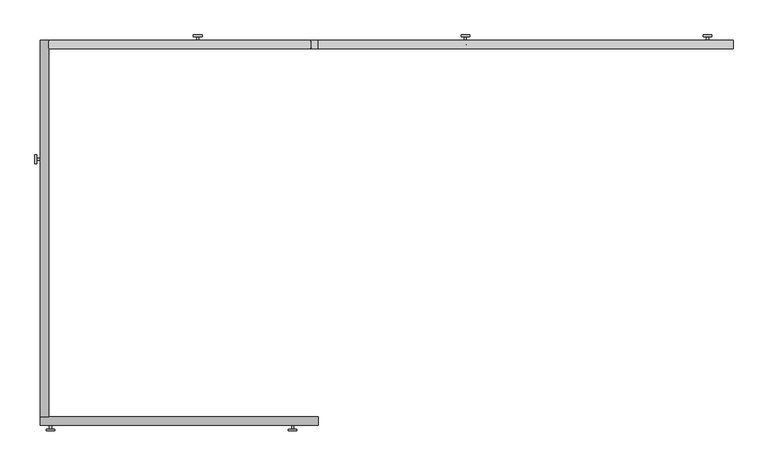
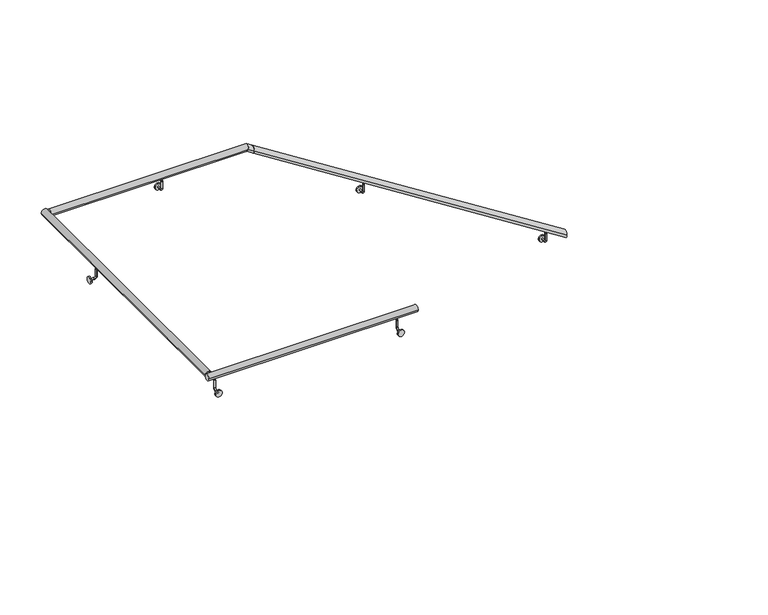
"""IFC4 building model written with IfcOpenShell, lengths in millimetres: railing geometry."""

from ifc_helpers import new_model, si_unit, point, frame, frame_2d, origin, place, context, project, spatial, circle_curve, ellipse_curve, trimmed, segment, composite_curve, outline, extrude, source, transform, mapped, element, save
from ifc_brep_helpers import plane_surface, cylinder_surface, revolved_surface, advanced_brep


def railing_9156e701(model_context):
    return source(origin(), model_context, "Body", "SolidModel", [
        advanced_brep(
        [(-47456.2877983, -5187.5461643, 4679.846421), (-47456.2877983, -5137.5461643, 4679.846421), (-49886.2877983, -5187.5461643, 6222.7035638), (-49886.2877983, -5137.5461643, 6222.7035638)],
        [
            (0, 1, ellipse_curve(frame((-47456.2877983, -5162.5461643, 4679.846421), z_axis=(1.0, 0.0, 0.0), x_axis=(0.0, 0.0, -1.0)), 29.613386, 25.0)),
            (1, 0, ellipse_curve(frame((-47456.2877983, -5162.5461643, 4679.846421), z_axis=(1.0, 0.0, 0.0), x_axis=(0.0, 0.0, -1.0)), 29.613386, 25.0)),
            (2, 3, ellipse_curve(frame((-49886.2877983, -5162.5461643, 6222.7035638), z_axis=(-1.0, 0.0, 0.0), x_axis=(0.0, 0.0, -1.0)), 29.613386, 25.0)),
            (3, 2, ellipse_curve(frame((-49886.2877983, -5162.5461643, 6222.7035638), z_axis=(-1.0, 0.0, 0.0), x_axis=(0.0, 0.0, -1.0)), 29.613386, 25.0)),
            (0, 2),
            (3, 1),
        ],
        [
            plane_surface(frame((-47456.2877983, -5162.5461643, 4709.459807), z_axis=(1.0, 0.0, 0.0), x_axis=(0.0, -1.0, 0.0))),
            plane_surface(frame((-49886.2877983, -5162.5461643, 6252.3169499), z_axis=(-1.0, 0.0, 0.0), x_axis=(0.0, -1.0, 0.0))),
            cylinder_surface(frame((-47469.6880017, -5162.5461643, 4688.3544866), z_axis=(0.8442128152478047, 0.0, -0.5360081366652713), x_axis=(0.0, 1.0, 0.0)), 25.0),
        ],
        [
            (0, [[1, 2]]),
            (1, [[3, 4]]),
            (2, [[-1, 5, -4, 6]]),
            (2, [[-2, -6, -3, -5]]),
        ],
    ),
        advanced_brep(
        [(-49886.2877983, -5187.5461643, 6222.7035638), (-49886.2877983, -5137.5461643, 6222.7035638), (-49933.6546852, -5187.5461643, 6252.7777778), (-49933.6546852, -5137.5461643, 6252.7777778), (-51463.5128792, -5187.5461643, 6252.7777778), (-51463.5128792, -5137.5461643, 6252.7777778)],
        [
            (0, 1, ellipse_curve(frame((-49886.2877983, -5162.5461643, 6222.7035638), z_axis=(1.0, 0.0, 0.0), x_axis=(0.0, 0.0, -1.0)), 29.613386, 25.0)),
            (1, 0, ellipse_curve(frame((-49886.2877983, -5162.5461643, 6222.7035638), z_axis=(1.0, 0.0, 0.0), x_axis=(0.0, 0.0, -1.0)), 29.613386, 25.0)),
            (0, 2),
            (2, 3, ellipse_curve(frame((-49933.6546852, -5162.5461643, 6252.7777778), z_axis=(0.9602637177483601, 0.0, -0.2790942356554467), x_axis=(-0.27909423565544716, 0.0, -0.9602637177483598)), 26.0345148, 25.0)),
            (3, 1),
            (3, 2, ellipse_curve(frame((-49933.6546852, -5162.5461643, 6252.7777778), z_axis=(0.9602637177483601, 0.0, -0.2790942356554467), x_axis=(-0.27909423565544716, 0.0, -0.9602637177483598)), 26.0345148, 25.0)),
            (4, 5, circle_curve(frame((-51463.5128792, -5162.5461643, 6252.7777778), z_axis=(-1.0, 0.0, 0.0), x_axis=(0.0, 1.0, 0.0)), 25.0)),
            (5, 4, circle_curve(frame((-51463.5128792, -5162.5461643, 6252.7777778), z_axis=(-1.0, 0.0, 0.0), x_axis=(0.0, 1.0, 0.0)), 25.0)),
            (2, 4),
            (5, 3),
        ],
        [
            plane_surface(frame((-49886.2877983, -5162.5461643, 6252.3169499), z_axis=(1.0, 0.0, 0.0), x_axis=(0.0, -1.0, 0.0))),
            cylinder_surface(frame((-49899.6880017, -5162.5461643, 6231.2116295), z_axis=(0.844212815247804, 0.0, -0.5360081366652724), x_axis=(0.0, 1.0, 0.0)), 25.0),
            plane_surface(frame((-51463.5128792, -5162.5461643, 6277.7777778), z_axis=(-1.0, 0.0, 0.0), x_axis=(0.0, -1.0, 0.0))),
            cylinder_surface(frame((-49926.3886022, -5162.5461643, 6252.7777778), z_axis=(1.0, 0.0, 0.0), x_axis=(0.0, 1.0, 0.0)), 25.0),
        ],
        [
            (0, [[1, 2]]),
            (1, [[-1, 3, 4, 5]]),
            (1, [[-2, -5, 6, -3]]),
            (2, [[7, 8]]),
            (3, [[-4, 9, -8, 10]]),
            (3, [[-6, -10, -7, -9]]),
        ],
    ),
        advanced_brep(
        [(-51463.5128792, -5137.5461643, 6252.7777778), (-51513.5128792, -5137.5461643, 6252.7777778), (-51463.5128792, -7342.3461643, 6252.7777778), (-51513.5128792, -7342.3461643, 6252.7777778)],
        [
            (0, 1, circle_curve(frame((-51488.5128792, -5137.5461643, 6252.7777778), z_axis=(0.0, 1.0, 0.0), x_axis=(-1.0, 0.0, 0.0)), 25.0)),
            (1, 0, circle_curve(frame((-51488.5128792, -5137.5461643, 6252.7777778), z_axis=(0.0, 1.0, 0.0), x_axis=(-1.0, 0.0, 0.0)), 25.0)),
            (2, 3, circle_curve(frame((-51488.5128792, -7342.3461643, 6252.7777778), z_axis=(0.0, -1.0, 0.0), x_axis=(-1.0, 0.0, 0.0)), 25.0)),
            (3, 2, circle_curve(frame((-51488.5128792, -7342.3461643, 6252.7777778), z_axis=(0.0, -1.0, 0.0), x_axis=(-1.0, 0.0, 0.0)), 25.0)),
            (0, 2),
            (3, 1),
        ],
        [
            plane_surface(frame((-51488.5128792, -5137.5461643, 6277.7777778), z_axis=(0.0, 1.0, 0.0), x_axis=(0.0, 0.0, -1.0))),
            plane_surface(frame((-51488.5128792, -7342.3461643, 6277.7777778), z_axis=(0.0, -1.0, 0.0), x_axis=(0.0, 0.0, -1.0))),
            cylinder_surface(frame((-51488.5128792, -5137.5461643, 6252.7777778), z_axis=(0.0, 1.0, 0.0), x_axis=(-1.0, 0.0, 0.0)), 25.0),
        ],
        [
            (0, [[1, 2]]),
            (1, [[3, 4]]),
            (2, [[-1, 5, -4, 6]]),
            (2, [[-2, -6, -3, -5]]),
        ],
    ),
        advanced_brep(
        [(-51513.5128792, -7342.3461643, 6252.7777778), (-51513.5128792, -7392.3461643, 6252.7777778), (-49886.2877983, -7342.3461643, 6252.7777778), (-49886.2877983, -7392.3461643, 6252.7777778)],
        [
            (0, 1, circle_curve(frame((-51513.5128792, -7367.3461643, 6252.7777778), z_axis=(-1.0, 0.0, 0.0), x_axis=(0.0, -1.0, 0.0)), 25.0)),
            (1, 0, circle_curve(frame((-51513.5128792, -7367.3461643, 6252.7777778), z_axis=(-1.0, 0.0, 0.0), x_axis=(0.0, -1.0, 0.0)), 25.0)),
            (2, 3, circle_curve(frame((-49886.2877983, -7367.3461643, 6252.7777778), z_axis=(1.0, 0.0, 0.0), x_axis=(0.0, -1.0, 0.0)), 25.0)),
            (3, 2, circle_curve(frame((-49886.2877983, -7367.3461643, 6252.7777778), z_axis=(1.0, 0.0, 0.0), x_axis=(0.0, -1.0, 0.0)), 25.0)),
            (0, 2),
            (3, 1),
        ],
        [
            plane_surface(frame((-51513.5128792, -7367.3461643, 6277.7777778), z_axis=(-1.0, 0.0, 0.0), x_axis=(0.0, 1.0, 0.0))),
            plane_surface(frame((-49886.2877983, -7367.3461643, 6277.7777778), z_axis=(1.0, 0.0, 0.0), x_axis=(0.0, 1.0, 0.0))),
            cylinder_surface(frame((-51513.5128792, -7367.3461643, 6252.7777778), z_axis=(-1.0, 0.0, 0.0), x_axis=(0.0, -1.0, 0.0)), 25.0),
        ],
        [
            (0, [[1, 2]]),
            (1, [[3, 4]]),
            (2, [[-1, 5, -4, 6]]),
            (2, [[-2, -6, -3, -5]]),
        ],
    ),
        advanced_brep(
        [(-51460.4878306, -7367.3461643, 6208.7277778), (-51447.7878306, -7367.3461643, 6208.7277778), (-51460.4878306, -7367.3461643, 6151.5777778), (-51447.7878306, -7367.3461643, 6151.5777778), (-51447.7878306, -7386.3961643, 6132.5277778), (-51460.4878306, -7386.3961643, 6132.5277778), (-51460.4878306, -7414.9711643, 6132.5277778), (-51447.7878306, -7414.9711643, 6132.5277778)],
        [
            (0, 1, circle_curve(frame((-51454.1378306, -7367.3461643, 6208.7277778), z_axis=(0.0, 0.0, 1.0), x_axis=(1.0, 0.0, 0.0)), 6.35)),
            (1, 0, circle_curve(frame((-51454.1378306, -7367.3461643, 6208.7277778), z_axis=(0.0, 0.0, 1.0), x_axis=(1.0, 0.0, 0.0)), 6.35)),
            (0, 2),
            (2, 3, circle_curve(frame((-51454.1378306, -7367.3461643, 6151.5777778), z_axis=(0.0, 0.0, 1.0), x_axis=(1.0, 0.0, 0.0)), 6.35)),
            (3, 1),
            (3, 2, circle_curve(frame((-51454.1378306, -7367.3461643, 6151.5777778), z_axis=(0.0, 0.0, 1.0), x_axis=(1.0, 0.0, 0.0)), 6.35)),
            (4, 3, circle_curve(frame((-51447.7878306, -7386.3961643, 6151.5777778), z_axis=(1.0, 0.0, 0.0), x_axis=(0.0, 1.0, 0.0)), 19.05)),
            (2, 5, circle_curve(frame((-51460.4878306, -7386.3961643, 6151.5777778), z_axis=(-1.0, 0.0, 0.0), x_axis=(0.0, 1.0, 0.0)), 19.05)),
            (5, 4, circle_curve(frame((-51454.1378306, -7386.3961643, 6132.5277778), z_axis=(0.0, 1.0, 0.0), x_axis=(1.0, 0.0, 0.0)), 6.35)),
            (4, 5, circle_curve(frame((-51454.1378306, -7386.3961643, 6132.5277778), z_axis=(0.0, 1.0, 0.0), x_axis=(1.0, 0.0, 0.0)), 6.35)),
            (6, 7, circle_curve(frame((-51454.1378306, -7414.9711643, 6132.5277778), z_axis=(0.0, -1.0, 0.0), x_axis=(1.0, 0.0, 0.0)), 6.35)),
            (7, 6, circle_curve(frame((-51454.1378306, -7414.9711643, 6132.5277778), z_axis=(0.0, -1.0, 0.0), x_axis=(1.0, 0.0, 0.0)), 6.35)),
            (5, 6),
            (7, 4),
        ],
        [
            plane_surface(frame((-51447.7878306, -7367.3461643, 6208.7277778), z_axis=(0.0, 0.0, 1.0), x_axis=(0.0, -1.0, 0.0))),
            cylinder_surface(frame((-51454.1378306, -7367.3461643, 6208.7277778), z_axis=(0.0, 0.0, 1.0), x_axis=(1.0, 0.0, 0.0)), 6.35),
            revolved_surface(trimmed(ellipse_curve(frame((-51454.1378306, -7367.3461643, 6151.5777778), z_axis=(0.0, 0.0, 1.0), x_axis=(1.0, 0.0, 0.0)), 6.35, 6.35), [point((-51460.4878306, -7367.3461643, 6151.5777778))], [point((-51447.7878306, -7367.3461643, 6151.5777778))], True, "CARTESIAN"), (-51454.1378306, -7386.3961643, 6151.5777778), (-1.0, 0.0, 0.0)),
            revolved_surface(trimmed(ellipse_curve(frame((-51454.1378306, -7367.3461643, 6151.5777778), z_axis=(0.0, 0.0, 1.0), x_axis=(1.0, 0.0, 0.0)), 6.35, 6.35), [point((-51447.7878306, -7367.3461643, 6151.5777778))], [point((-51460.4878306, -7367.3461643, 6151.5777778))], True, "CARTESIAN"), (-51454.1378306, -7386.3961643, 6151.5777778), (-1.0, 0.0, 0.0)),
            plane_surface(frame((-51454.1378306, -7414.9711643, 6126.1777778), z_axis=(0.0, -1.0, 0.0), x_axis=(1.0, 0.0, 0.0))),
            cylinder_surface(frame((-51454.1378306, -7386.3961643, 6132.5277778), z_axis=(0.0, 1.0, 0.0), x_axis=(1.0, 0.0, 0.0)), 6.35),
        ],
        [
            (0, [[1, 2]]),
            (1, [[-1, 3, 4, 5]]),
            (1, [[-2, -5, 6, -3]]),
            (2, [[7, -4, 8, 9]]),
            (3, [[-8, -6, -7, 10]]),
            (4, [[11, 12]]),
            (5, [[-9, 13, -12, 14]]),
            (5, [[-10, -14, -11, -13]]),
        ],
    ),
        extrude(outline(composite_curve([segment(trimmed(circle_curve(frame_2d((6132.5277778, -51454.1378306)), 25.4), [point((6132.5277778, -51428.7378306))], [point((6132.5277778, -51479.5378306))], False, "CARTESIAN"), True, "CONTINUOUS"), segment(trimmed(circle_curve(frame_2d((6132.5277778, -51454.1378306)), 25.4), [point((6132.5277778, -51479.5378306))], [point((6132.5277778, -51428.7378306))], False, "CARTESIAN"), True, "CONTINUOUS")], self_intersect=False)), frame((0.0, -7424.4961643, 0.0), z_axis=(0.0, 1.0, 0.0), x_axis=(0.0, 0.0, 1.0)), (0.0, 0.0, 1.0), 9.525),
        advanced_brep(
        [(-51488.5128792, -5827.5211804, 6208.7277778), (-51488.5128792, -5840.2211804, 6208.7277778), (-51488.5128792, -5827.5211804, 6151.5777778), (-51488.5128792, -5840.2211804, 6151.5777778), (-51507.5628792, -5840.2211804, 6132.5277778), (-51507.5628792, -5827.5211804, 6132.5277778), (-51536.1378792, -5827.5211804, 6132.5277778), (-51536.1378792, -5840.2211804, 6132.5277778)],
        [
            (0, 1, circle_curve(frame((-51488.5128792, -5833.8711804, 6208.7277778), z_axis=(0.0, 0.0, 1.0), x_axis=(0.0, -1.0, 0.0)), 6.35)),
            (1, 0, circle_curve(frame((-51488.5128792, -5833.8711804, 6208.7277778), z_axis=(0.0, 0.0, 1.0), x_axis=(0.0, -1.0, 0.0)), 6.35)),
            (0, 2),
            (2, 3, circle_curve(frame((-51488.5128792, -5833.8711804, 6151.5777778), z_axis=(0.0, 0.0, 1.0), x_axis=(0.0, -1.0, 0.0)), 6.35)),
            (3, 1),
            (3, 2, circle_curve(frame((-51488.5128792, -5833.8711804, 6151.5777778), z_axis=(0.0, 0.0, 1.0), x_axis=(0.0, -1.0, 0.0)), 6.35)),
            (4, 3, circle_curve(frame((-51507.5628792, -5840.2211804, 6151.5777778), z_axis=(0.0, -1.0, 0.0), x_axis=(1.0, 0.0, 0.0)), 19.05)),
            (2, 5, circle_curve(frame((-51507.5628792, -5827.5211804, 6151.5777778), z_axis=(0.0, 1.0, 0.0), x_axis=(1.0, 0.0, 0.0)), 19.05)),
            (5, 4, circle_curve(frame((-51507.5628792, -5833.8711804, 6132.5277778), z_axis=(1.0, 0.0, 0.0), x_axis=(0.0, -1.0, 0.0)), 6.35)),
            (4, 5, circle_curve(frame((-51507.5628792, -5833.8711804, 6132.5277778), z_axis=(1.0, 0.0, 0.0), x_axis=(0.0, -1.0, 0.0)), 6.35)),
            (6, 7, circle_curve(frame((-51536.1378792, -5833.8711804, 6132.5277778), z_axis=(-1.0, 0.0, 0.0), x_axis=(0.0, -1.0, 0.0)), 6.35)),
            (7, 6, circle_curve(frame((-51536.1378792, -5833.8711804, 6132.5277778), z_axis=(-1.0, 0.0, 0.0), x_axis=(0.0, -1.0, 0.0)), 6.35)),
            (5, 6),
            (7, 4),
        ],
        [
            plane_surface(frame((-51488.5128792, -5840.2211804, 6208.7277778), z_axis=(0.0, 0.0, 1.0), x_axis=(-1.0, 0.0, 0.0))),
            cylinder_surface(frame((-51488.5128792, -5833.8711804, 6208.7277778), z_axis=(0.0, 0.0, 1.0), x_axis=(0.0, -1.0, 0.0)), 6.35),
            revolved_surface(trimmed(ellipse_curve(frame((-51488.5128792, -5833.8711804, 6151.5777778), z_axis=(0.0, 0.0, 1.0), x_axis=(0.0, -1.0, 0.0)), 6.35, 6.35), [point((-51488.5128792, -5827.5211804, 6151.5777778))], [point((-51488.5128792, -5840.2211804, 6151.5777778))], True, "CARTESIAN"), (-51507.5628792, -5833.8711804, 6151.5777778), (0.0, 1.0, 0.0)),
            revolved_surface(trimmed(ellipse_curve(frame((-51488.5128792, -5833.8711804, 6151.5777778), z_axis=(0.0, 0.0, 1.0), x_axis=(0.0, -1.0, 0.0)), 6.35, 6.35), [point((-51488.5128792, -5840.2211804, 6151.5777778))], [point((-51488.5128792, -5827.5211804, 6151.5777778))], True, "CARTESIAN"), (-51507.5628792, -5833.8711804, 6151.5777778), (0.0, 1.0, 0.0)),
            plane_surface(frame((-51536.1378792, -5833.8711804, 6126.1777778), z_axis=(-1.0, 0.0, 0.0), x_axis=(0.0, -1.0, 0.0))),
            cylinder_surface(frame((-51507.5628792, -5833.8711804, 6132.5277778), z_axis=(1.0, 0.0, 0.0), x_axis=(0.0, -1.0, 0.0)), 6.35),
        ],
        [
            (0, [[1, 2]]),
            (1, [[-1, 3, 4, 5]]),
            (1, [[-2, -5, 6, -3]]),
            (2, [[7, -4, 8, 9]]),
            (3, [[-8, -6, -7, 10]]),
            (4, [[11, 12]]),
            (5, [[-9, 13, -12, 14]]),
            (5, [[-10, -14, -11, -13]]),
        ],
    ),
        extrude(outline(composite_curve([segment(trimmed(circle_curve(frame_2d((-5833.8711804, 6132.5277778)), 25.4), [point((-5859.2711804, 6132.5277778))], [point((-5808.4711804, 6132.5277778))], False, "CARTESIAN"), True, "CONTINUOUS"), segment(trimmed(circle_curve(frame_2d((-5833.8711804, 6132.5277778)), 25.4), [point((-5808.4711804, 6132.5277778))], [point((-5859.2711804, 6132.5277778))], False, "CARTESIAN"), True, "CONTINUOUS")], self_intersect=False)), frame((-51545.6628792, 0.0, 0.0), z_axis=(1.0, 0.0, 0.0), x_axis=(0.0, 1.0, 0.0)), (0.0, 0.0, 1.0), 9.525),
        advanced_brep(
        [(-50585.637863, -5162.5461643, 6208.7277778), (-50598.337863, -5162.5461643, 6208.7277778), (-50585.637863, -5162.5461643, 6151.5777778), (-50598.337863, -5162.5461643, 6151.5777778), (-50598.337863, -5143.4961643, 6132.5277778), (-50585.637863, -5143.4961643, 6132.5277778), (-50585.637863, -5114.9211643, 6132.5277778), (-50598.337863, -5114.9211643, 6132.5277778)],
        [
            (0, 1, circle_curve(frame((-50591.987863, -5162.5461643, 6208.7277778), z_axis=(0.0, 0.0, 1.0), x_axis=(-1.0, 0.0, 0.0)), 6.35)),
            (1, 0, circle_curve(frame((-50591.987863, -5162.5461643, 6208.7277778), z_axis=(0.0, 0.0, 1.0), x_axis=(-1.0, 0.0, 0.0)), 6.35)),
            (0, 2),
            (2, 3, circle_curve(frame((-50591.987863, -5162.5461643, 6151.5777778), z_axis=(0.0, 0.0, 1.0), x_axis=(-1.0, 0.0, 0.0)), 6.35)),
            (3, 1),
            (3, 2, circle_curve(frame((-50591.987863, -5162.5461643, 6151.5777778), z_axis=(0.0, 0.0, 1.0), x_axis=(-1.0, 0.0, 0.0)), 6.35)),
            (4, 3, circle_curve(frame((-50598.337863, -5143.4961643, 6151.5777778), z_axis=(-1.0, 0.0, 0.0), x_axis=(0.0, -1.0, 0.0)), 19.05)),
            (2, 5, circle_curve(frame((-50585.637863, -5143.4961643, 6151.5777778), z_axis=(1.0, 0.0, 0.0), x_axis=(0.0, -1.0, 0.0)), 19.05)),
            (5, 4, circle_curve(frame((-50591.987863, -5143.4961643, 6132.5277778), z_axis=(0.0, -1.0, 0.0), x_axis=(-1.0, 0.0, 0.0)), 6.35)),
            (4, 5, circle_curve(frame((-50591.987863, -5143.4961643, 6132.5277778), z_axis=(0.0, -1.0, 0.0), x_axis=(-1.0, 0.0, 0.0)), 6.35)),
            (6, 7, circle_curve(frame((-50591.987863, -5114.9211643, 6132.5277778), z_axis=(0.0, 1.0, 0.0), x_axis=(-1.0, 0.0, 0.0)), 6.35)),
            (7, 6, circle_curve(frame((-50591.987863, -5114.9211643, 6132.5277778), z_axis=(0.0, 1.0, 0.0), x_axis=(-1.0, 0.0, 0.0)), 6.35)),
            (5, 6),
            (7, 4),
        ],
        [
            plane_surface(frame((-50598.337863, -5162.5461643, 6208.7277778), z_axis=(0.0, 0.0, 1.0), x_axis=(0.0, 1.0, 0.0))),
            cylinder_surface(frame((-50591.987863, -5162.5461643, 6208.7277778), z_axis=(0.0, 0.0, 1.0), x_axis=(-1.0, 0.0, 0.0)), 6.35),
            revolved_surface(trimmed(ellipse_curve(frame((-50591.987863, -5162.5461643, 6151.5777778), z_axis=(0.0, 0.0, 1.0), x_axis=(-1.0, 0.0, 0.0)), 6.35, 6.35), [point((-50585.637863, -5162.5461643, 6151.5777778))], [point((-50598.337863, -5162.5461643, 6151.5777778))], True, "CARTESIAN"), (-50591.987863, -5143.4961643, 6151.5777778), (1.0, 0.0, 0.0)),
            revolved_surface(trimmed(ellipse_curve(frame((-50591.987863, -5162.5461643, 6151.5777778), z_axis=(0.0, 0.0, 1.0), x_axis=(-1.0, 0.0, 0.0)), 6.35, 6.35), [point((-50598.337863, -5162.5461643, 6151.5777778))], [point((-50585.637863, -5162.5461643, 6151.5777778))], True, "CARTESIAN"), (-50591.987863, -5143.4961643, 6151.5777778), (1.0, 0.0, 0.0)),
            plane_surface(frame((-50591.987863, -5114.9211643, 6126.1777778), z_axis=(0.0, 1.0, 0.0), x_axis=(-1.0, 0.0, 0.0))),
            cylinder_surface(frame((-50591.987863, -5143.4961643, 6132.5277778), z_axis=(0.0, -1.0, 0.0), x_axis=(-1.0, 0.0, 0.0)), 6.35),
        ],
        [
            (0, [[1, 2]]),
            (1, [[-1, 3, 4, 5]]),
            (1, [[-2, -5, 6, -3]]),
            (2, [[7, -4, 8, 9]]),
            (3, [[-8, -6, -7, 10]]),
            (4, [[11, 12]]),
            (5, [[-9, 13, -12, 14]]),
            (5, [[-10, -14, -11, -13]]),
        ],
    ),
        extrude(outline(composite_curve([segment(trimmed(circle_curve(frame_2d((6132.5277778, -50591.987863)), 25.4), [point((6132.5277778, -50617.387863))], [point((6132.5277778, -50566.587863))], False, "CARTESIAN"), True, "CONTINUOUS"), segment(trimmed(circle_curve(frame_2d((6132.5277778, -50591.987863)), 25.4), [point((6132.5277778, -50566.587863))], [point((6132.5277778, -50617.387863))], False, "CARTESIAN"), True, "CONTINUOUS")], self_intersect=False)), frame((0.0, -5114.9211643, 0.0), z_axis=(0.0, 1.0, 0.0), x_axis=(0.0, 0.0, 1.0)), (0.0, 0.0, 1.0), 9.525),
        advanced_brep(
        [(-49017.7878306, -5162.5461643, 5635.870145), (-49030.4878306, -5162.5461643, 5635.870145), (-49017.7878306, -5162.5461643, 5578.720145), (-49030.4878306, -5162.5461643, 5578.720145), (-49030.4878306, -5143.4961643, 5559.670145), (-49017.7878306, -5143.4961643, 5559.670145), (-49017.7878306, -5114.9211643, 5559.670145), (-49030.4878306, -5114.9211643, 5559.670145)],
        [
            (0, 1, circle_curve(frame((-49024.1378306, -5162.5461643, 5635.870145), z_axis=(0.0, 0.0, 1.0), x_axis=(-1.0, 0.0, 0.0)), 6.35)),
            (1, 0, circle_curve(frame((-49024.1378306, -5162.5461643, 5635.870145), z_axis=(0.0, 0.0, 1.0), x_axis=(-1.0, 0.0, 0.0)), 6.35)),
            (0, 2),
            (2, 3, circle_curve(frame((-49024.1378306, -5162.5461643, 5578.720145), z_axis=(0.0, 0.0, 1.0), x_axis=(-1.0, 0.0, 0.0)), 6.35)),
            (3, 1),
            (3, 2, circle_curve(frame((-49024.1378306, -5162.5461643, 5578.720145), z_axis=(0.0, 0.0, 1.0), x_axis=(-1.0, 0.0, 0.0)), 6.35)),
            (4, 3, circle_curve(frame((-49030.4878306, -5143.4961643, 5578.720145), z_axis=(-1.0, 0.0, 0.0), x_axis=(0.0, -1.0, 0.0)), 19.05)),
            (2, 5, circle_curve(frame((-49017.7878306, -5143.4961643, 5578.720145), z_axis=(1.0, 0.0, 0.0), x_axis=(0.0, -1.0, 0.0)), 19.05)),
            (5, 4, circle_curve(frame((-49024.1378306, -5143.4961643, 5559.670145), z_axis=(0.0, -1.0, 0.0), x_axis=(-1.0, 0.0, 0.0)), 6.35)),
            (4, 5, circle_curve(frame((-49024.1378306, -5143.4961643, 5559.670145), z_axis=(0.0, -1.0, 0.0), x_axis=(-1.0, 0.0, 0.0)), 6.35)),
            (6, 7, circle_curve(frame((-49024.1378306, -5114.9211643, 5559.670145), z_axis=(0.0, 1.0, 0.0), x_axis=(-1.0, 0.0, 0.0)), 6.35)),
            (7, 6, circle_curve(frame((-49024.1378306, -5114.9211643, 5559.670145), z_axis=(0.0, 1.0, 0.0), x_axis=(-1.0, 0.0, 0.0)), 6.35)),
            (5, 6),
            (7, 4),
        ],
        [
            plane_surface(frame((-49030.4878306, -5162.5461643, 5635.870145), z_axis=(0.0, 0.0, 1.0), x_axis=(0.0, 1.0, 0.0))),
            cylinder_surface(frame((-49024.1378306, -5162.5461643, 5635.870145), z_axis=(0.0, 0.0, 1.0), x_axis=(-1.0, 0.0, 0.0)), 6.35),
            revolved_surface(trimmed(ellipse_curve(frame((-49024.1378306, -5162.5461643, 5578.720145), z_axis=(0.0, 0.0, 1.0), x_axis=(-1.0, 0.0, 0.0)), 6.35, 6.35), [point((-49017.7878306, -5162.5461643, 5578.720145))], [point((-49030.4878306, -5162.5461643, 5578.720145))], True, "CARTESIAN"), (-49024.1378306, -5143.4961643, 5578.720145), (1.0, 0.0, 0.0)),
            revolved_surface(trimmed(ellipse_curve(frame((-49024.1378306, -5162.5461643, 5578.720145), z_axis=(0.0, 0.0, 1.0), x_axis=(-1.0, 0.0, 0.0)), 6.35, 6.35), [point((-49030.4878306, -5162.5461643, 5578.720145))], [point((-49017.7878306, -5162.5461643, 5578.720145))], True, "CARTESIAN"), (-49024.1378306, -5143.4961643, 5578.720145), (1.0, 0.0, 0.0)),
            plane_surface(frame((-49024.1378306, -5114.9211643, 5553.320145), z_axis=(0.0, 1.0, 0.0), x_axis=(-1.0, 0.0, 0.0))),
            cylinder_surface(frame((-49024.1378306, -5143.4961643, 5559.670145), z_axis=(0.0, -1.0, 0.0), x_axis=(-1.0, 0.0, 0.0)), 6.35),
        ],
        [
            (0, [[1, 2]]),
            (1, [[-1, 3, 4, 5]]),
            (1, [[-2, -5, 6, -3]]),
            (2, [[7, -4, 8, 9]]),
            (3, [[-8, -6, -7, 10]]),
            (4, [[11, 12]]),
            (5, [[-9, 13, -12, 14]]),
            (5, [[-10, -14, -11, -13]]),
        ],
    ),
        extrude(outline(composite_curve([segment(trimmed(circle_curve(frame_2d((5559.670145, -49024.1378306)), 25.4), [point((5559.670145, -49049.5378306))], [point((5559.670145, -48998.7378306))], False, "CARTESIAN"), True, "CONTINUOUS"), segment(trimmed(circle_curve(frame_2d((5559.670145, -49024.1378306)), 25.4), [point((5559.670145, -48998.7378306))], [point((5559.670145, -49049.5378306))], False, "CARTESIAN"), True, "CONTINUOUS")], self_intersect=False)), frame((0.0, -5114.9211643, 0.0), z_axis=(0.0, 1.0, 0.0), x_axis=(0.0, 0.0, 1.0)), (0.0, 0.0, 1.0), 9.525),
        advanced_brep(
        [(-50042.6377983, -7367.3461643, 6208.7277778), (-50029.9377983, -7367.3461643, 6208.7277778), (-50042.6377983, -7367.3461643, 6151.5777778), (-50029.9377983, -7367.3461643, 6151.5777778), (-50029.9377983, -7386.3961643, 6132.5277778), (-50042.6377983, -7386.3961643, 6132.5277778), (-50042.6377983, -7414.9711643, 6132.5277778), (-50029.9377983, -7414.9711643, 6132.5277778)],
        [
            (0, 1, circle_curve(frame((-50036.2877983, -7367.3461643, 6208.7277778), z_axis=(0.0, 0.0, 1.0), x_axis=(1.0, 0.0, 0.0)), 6.35)),
            (1, 0, circle_curve(frame((-50036.2877983, -7367.3461643, 6208.7277778), z_axis=(0.0, 0.0, 1.0), x_axis=(1.0, 0.0, 0.0)), 6.35)),
            (0, 2),
            (2, 3, circle_curve(frame((-50036.2877983, -7367.3461643, 6151.5777778), z_axis=(0.0, 0.0, 1.0), x_axis=(1.0, 0.0, 0.0)), 6.35)),
            (3, 1),
            (3, 2, circle_curve(frame((-50036.2877983, -7367.3461643, 6151.5777778), z_axis=(0.0, 0.0, 1.0), x_axis=(1.0, 0.0, 0.0)), 6.35)),
            (4, 3, circle_curve(frame((-50029.9377983, -7386.3961643, 6151.5777778), z_axis=(1.0, 0.0, 0.0), x_axis=(0.0, 1.0, 0.0)), 19.05)),
            (2, 5, circle_curve(frame((-50042.6377983, -7386.3961643, 6151.5777778), z_axis=(-1.0, 0.0, 0.0), x_axis=(0.0, 1.0, 0.0)), 19.05)),
            (5, 4, circle_curve(frame((-50036.2877983, -7386.3961643, 6132.5277778), z_axis=(0.0, 1.0, 0.0), x_axis=(1.0, 0.0, 0.0)), 6.35)),
            (4, 5, circle_curve(frame((-50036.2877983, -7386.3961643, 6132.5277778), z_axis=(0.0, 1.0, 0.0), x_axis=(1.0, 0.0, 0.0)), 6.35)),
            (6, 7, circle_curve(frame((-50036.2877983, -7414.9711643, 6132.5277778), z_axis=(0.0, -1.0, 0.0), x_axis=(1.0, 0.0, 0.0)), 6.35)),
            (7, 6, circle_curve(frame((-50036.2877983, -7414.9711643, 6132.5277778), z_axis=(0.0, -1.0, 0.0), x_axis=(1.0, 0.0, 0.0)), 6.35)),
            (5, 6),
            (7, 4),
        ],
        [
            plane_surface(frame((-50029.9377983, -7367.3461643, 6208.7277778), z_axis=(0.0, 0.0, 1.0), x_axis=(0.0, -1.0, 0.0))),
            cylinder_surface(frame((-50036.2877983, -7367.3461643, 6208.7277778), z_axis=(0.0, 0.0, 1.0), x_axis=(1.0, 0.0, 0.0)), 6.35),
            revolved_surface(trimmed(ellipse_curve(frame((-50036.2877983, -7367.3461643, 6151.5777778), z_axis=(0.0, 0.0, 1.0), x_axis=(1.0, 0.0, 0.0)), 6.35, 6.35), [point((-50042.6377983, -7367.3461643, 6151.5777778))], [point((-50029.9377983, -7367.3461643, 6151.5777778))], True, "CARTESIAN"), (-50036.2877983, -7386.3961643, 6151.5777778), (-1.0, 0.0, 0.0)),
            revolved_surface(trimmed(ellipse_curve(frame((-50036.2877983, -7367.3461643, 6151.5777778), z_axis=(0.0, 0.0, 1.0), x_axis=(1.0, 0.0, 0.0)), 6.35, 6.35), [point((-50029.9377983, -7367.3461643, 6151.5777778))], [point((-50042.6377983, -7367.3461643, 6151.5777778))], True, "CARTESIAN"), (-50036.2877983, -7386.3961643, 6151.5777778), (-1.0, 0.0, 0.0)),
            plane_surface(frame((-50036.2877983, -7414.9711643, 6126.1777778), z_axis=(0.0, -1.0, 0.0), x_axis=(1.0, 0.0, 0.0))),
            cylinder_surface(frame((-50036.2877983, -7386.3961643, 6132.5277778), z_axis=(0.0, 1.0, 0.0), x_axis=(1.0, 0.0, 0.0)), 6.35),
        ],
        [
            (0, [[1, 2]]),
            (1, [[-1, 3, 4, 5]]),
            (1, [[-2, -5, 6, -3]]),
            (2, [[7, -4, 8, 9]]),
            (3, [[-8, -6, -7, 10]]),
            (4, [[11, 12]]),
            (5, [[-9, 13, -12, 14]]),
            (5, [[-10, -14, -11, -13]]),
        ],
    ),
        extrude(outline(composite_curve([segment(trimmed(circle_curve(frame_2d((6132.5277778, -50036.2877983)), 25.4), [point((6132.5277778, -50010.8877983))], [point((6132.5277778, -50061.6877983))], False, "CARTESIAN"), True, "CONTINUOUS"), segment(trimmed(circle_curve(frame_2d((6132.5277778, -50036.2877983)), 25.4), [point((6132.5277778, -50061.6877983))], [point((6132.5277778, -50010.8877983))], False, "CARTESIAN"), True, "CONTINUOUS")], self_intersect=False)), frame((0.0, -7424.4961643, 0.0), z_axis=(0.0, 1.0, 0.0), x_axis=(0.0, 0.0, 1.0)), (0.0, 0.0, 1.0), 9.525),
        advanced_brep(
        [(-47599.9377983, -5162.5461643, 4735.6479023), (-47612.6377983, -5162.5461643, 4735.6479023), (-47599.9377983, -5162.5461643, 4678.4979023), (-47612.6377983, -5162.5461643, 4678.4979023), (-47612.6377983, -5143.4961643, 4659.4479023), (-47599.9377983, -5143.4961643, 4659.4479023), (-47599.9377983, -5114.9211643, 4659.4479023), (-47612.6377983, -5114.9211643, 4659.4479023)],
        [
            (0, 1, circle_curve(frame((-47606.2877983, -5162.5461643, 4735.6479023), z_axis=(0.0, 0.0, 1.0), x_axis=(-1.0, 0.0, 0.0)), 6.35)),
            (1, 0, circle_curve(frame((-47606.2877983, -5162.5461643, 4735.6479023), z_axis=(0.0, 0.0, 1.0), x_axis=(-1.0, 0.0, 0.0)), 6.35)),
            (0, 2),
            (2, 3, circle_curve(frame((-47606.2877983, -5162.5461643, 4678.4979023), z_axis=(0.0, 0.0, 1.0), x_axis=(-1.0, 0.0, 0.0)), 6.35)),
            (3, 1),
            (3, 2, circle_curve(frame((-47606.2877983, -5162.5461643, 4678.4979023), z_axis=(0.0, 0.0, 1.0), x_axis=(-1.0, 0.0, 0.0)), 6.35)),
            (4, 3, circle_curve(frame((-47612.6377983, -5143.4961643, 4678.4979023), z_axis=(-1.0, 0.0, 0.0), x_axis=(0.0, -1.0, 0.0)), 19.05)),
            (2, 5, circle_curve(frame((-47599.9377983, -5143.4961643, 4678.4979023), z_axis=(1.0, 0.0, 0.0), x_axis=(0.0, -1.0, 0.0)), 19.05)),
            (5, 4, circle_curve(frame((-47606.2877983, -5143.4961643, 4659.4479023), z_axis=(0.0, -1.0, 0.0), x_axis=(-1.0, 0.0, 0.0)), 6.35)),
            (4, 5, circle_curve(frame((-47606.2877983, -5143.4961643, 4659.4479023), z_axis=(0.0, -1.0, 0.0), x_axis=(-1.0, 0.0, 0.0)), 6.35)),
            (6, 7, circle_curve(frame((-47606.2877983, -5114.9211643, 4659.4479023), z_axis=(0.0, 1.0, 0.0), x_axis=(-1.0, 0.0, 0.0)), 6.35)),
            (7, 6, circle_curve(frame((-47606.2877983, -5114.9211643, 4659.4479023), z_axis=(0.0, 1.0, 0.0), x_axis=(-1.0, 0.0, 0.0)), 6.35)),
            (5, 6),
            (7, 4),
        ],
        [
            plane_surface(frame((-47612.6377983, -5162.5461643, 4735.6479023), z_axis=(0.0, 0.0, 1.0), x_axis=(0.0, 1.0, 0.0))),
            cylinder_surface(frame((-47606.2877983, -5162.5461643, 4735.6479023), z_axis=(0.0, 0.0, 1.0), x_axis=(-1.0, 0.0, 0.0)), 6.35),
            revolved_surface(trimmed(ellipse_curve(frame((-47606.2877983, -5162.5461643, 4678.4979023), z_axis=(0.0, 0.0, 1.0), x_axis=(-1.0, 0.0, 0.0)), 6.35, 6.35), [point((-47599.9377983, -5162.5461643, 4678.4979023))], [point((-47612.6377983, -5162.5461643, 4678.4979023))], True, "CARTESIAN"), (-47606.2877983, -5143.4961643, 4678.4979023), (1.0, 0.0, 0.0)),
            revolved_surface(trimmed(ellipse_curve(frame((-47606.2877983, -5162.5461643, 4678.4979023), z_axis=(0.0, 0.0, 1.0), x_axis=(-1.0, 0.0, 0.0)), 6.35, 6.35), [point((-47612.6377983, -5162.5461643, 4678.4979023))], [point((-47599.9377983, -5162.5461643, 4678.4979023))], True, "CARTESIAN"), (-47606.2877983, -5143.4961643, 4678.4979023), (1.0, 0.0, 0.0)),
            plane_surface(frame((-47606.2877983, -5114.9211643, 4653.0979023), z_axis=(0.0, 1.0, 0.0), x_axis=(-1.0, 0.0, 0.0))),
            cylinder_surface(frame((-47606.2877983, -5143.4961643, 4659.4479023), z_axis=(0.0, -1.0, 0.0), x_axis=(-1.0, 0.0, 0.0)), 6.35),
        ],
        [
            (0, [[1, 2]]),
            (1, [[-1, 3, 4, 5]]),
            (1, [[-2, -5, 6, -3]]),
            (2, [[7, -4, 8, 9]]),
            (3, [[-8, -6, -7, 10]]),
            (4, [[11, 12]]),
            (5, [[-9, 13, -12, 14]]),
            (5, [[-10, -14, -11, -13]]),
        ],
    ),
        extrude(outline(composite_curve([segment(trimmed(circle_curve(frame_2d((4659.4479023, -47606.2877983)), 25.4), [point((4659.4479023, -47631.6877983))], [point((4659.4479023, -47580.8877983))], False, "CARTESIAN"), True, "CONTINUOUS"), segment(trimmed(circle_curve(frame_2d((4659.4479023, -47606.2877983)), 25.4), [point((4659.4479023, -47580.8877983))], [point((4659.4479023, -47631.6877983))], False, "CARTESIAN"), True, "CONTINUOUS")], self_intersect=False)), frame((0.0, -5114.9211643, 0.0), z_axis=(0.0, 1.0, 0.0), x_axis=(0.0, 0.0, 1.0)), (0.0, 0.0, 1.0), 9.525),
    ])


if __name__ == "__main__":
    model = new_model("IFC4")
    model_context = context("Model", 3, world=origin())
    ifc_project = project(units=[si_unit("LENGTHUNIT", "METRE", prefix="MILLI")], contexts=[model_context])
    site = spatial("IfcSite", under=ifc_project)
    building = spatial("IfcBuilding", under=site)
    placement = place(None, origin())
    railing_shape = railing_9156e701(model_context)
    element("IfcRailing", 1, at=placement, inside=building, context=model_context, shape_type="MappedRepresentation", body=[
        mapped(railing_shape, transform((0.0, 0.0, 0.0), x_axis=(1.0, 0.0, 0.0), y_axis=(0.0, 1.0, 0.0), z_axis=(0.0, 0.0, 1.0))),
    ])
    save(model, "model.ifc")
